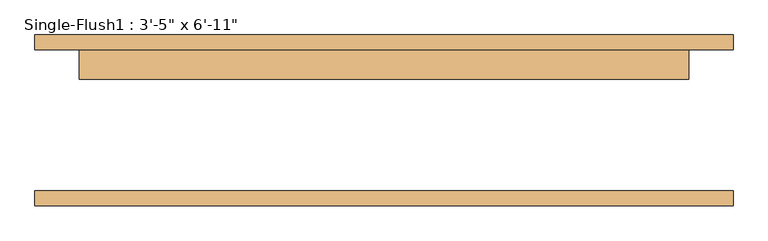
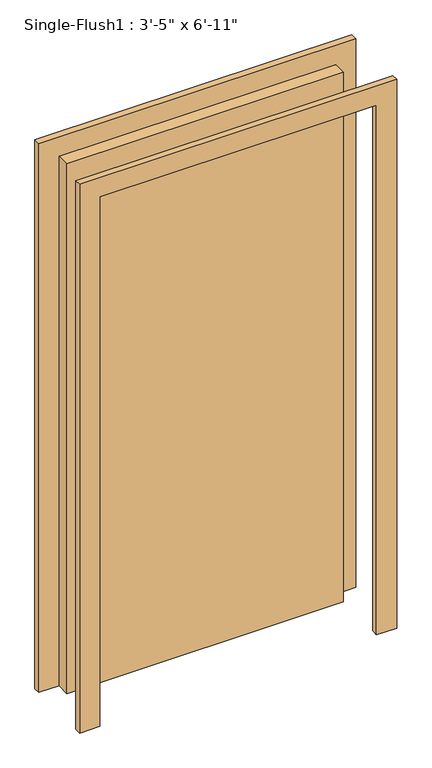
"""IFC4 building model written with IfcOpenShell, lengths in millimetres: door geometry."""

from ifc_helpers import new_model, si_unit, frame, origin, origin_with_axes, place, context, project, spatial, polyline, outline, extrude, source, transform, mapped, element, save


def door_eaa92909(model_context):
    return source(origin(), model_context, "Body", "SweptSolid", [
        extrude(outline(polyline([(2184.4, -596.9), (0.0, -596.9), (0.0, -520.7), (2108.2, -520.7), (2108.2, 520.7), (0.0, 520.7), (0.0, 596.9), (2184.4, 596.9), (2184.4, -596.9)])), frame((0.0, 120.65, 0.0), z_axis=(0.0, 1.0, 0.0), x_axis=(0.0, 0.0, 1.0)), (0.0, 0.0, 1.0), 25.4),
        extrude(outline(polyline([(2184.4, 596.9), (2184.4, -596.9), (0.0, -596.9), (0.0, -520.7), (2108.2, -520.7), (2108.2, 520.7), (0.0, 520.7), (0.0, 596.9), (2184.4, 596.9)])), frame((0.0, -146.05, 0.0), z_axis=(0.0, 1.0, 0.0), x_axis=(0.0, 0.0, 1.0)), (0.0, 0.0, 1.0), 25.4),
        extrude(outline(polyline([(520.7, 69.85), (-520.7, 69.85), (-520.7, 120.65), (520.7, 120.65), (520.7, 69.85)])), origin_with_axes(), (0.0, 0.0, 1.0), 2108.2),
    ])


if __name__ == "__main__":
    model = new_model("IFC4")
    model_context = context("Model", 3, world=origin())
    ifc_project = project(units=[si_unit("LENGTHUNIT", "METRE", prefix="MILLI")], contexts=[model_context])
    site = spatial("IfcSite", under=ifc_project)
    building = spatial("IfcBuilding", under=site)
    placement = place(None, origin())
    door_shape = door_eaa92909(model_context)
    element("IfcDoor", 1, ObjectType="Single-Flush1 : 3'-5\" x 6'-11\"", at=placement, inside=building, context=model_context, shape_type="MappedRepresentation", body=[
        mapped(door_shape, transform((0.0, 0.0, 0.0), x_axis=(1.0, 0.0, 0.0), y_axis=(0.0, 1.0, 0.0), z_axis=(0.0, 0.0, 1.0))),
    ])
    save(model, "model.ifc")

# Revit data of these elements
# Type "Single-Flush1 : 3'-5\" x 6'-11\""
#   Type Mark = "21"
#   Construction Type Id = "MDOOR"
#   Assembly Code = "C1020"
#   Analytic Construction = "Metal"
#   Thickness = 0' - 2"
#   Heat Transfer Coefficient (U) = 3.7021 W/(m²·K)
#   Height = 6' - 11"
#   Trim Projection Ext = 0' - 1"
#   Trim Projection Int = 0' - 1"
#   Trim Width = 0' - 3"
#   Width = 3' - 5"
#   Door Material = Door - Panel
#   Frame Material = Door - Frame
#   Visual Light Transmittance = 0
#   Solar Heat Gain Coefficient = 0
#   Function = (empty or 0)
#   Wall Closure = (empty or 0)
# Element 1 (IfcDoor, "Single-Flush1 : 3'-5\" x 6'-11\"")
#   Materials on its faces: "Door - Frame", "Door - Panel"
# Materials
#   "Door - Panel": class "Wood", colour RGB 210 159 95, transparency 0, Cost = 0
#   "Door - Frame": class "Miscellaneous", colour RGB 118 70 51, transparency 0, Cost = 0
